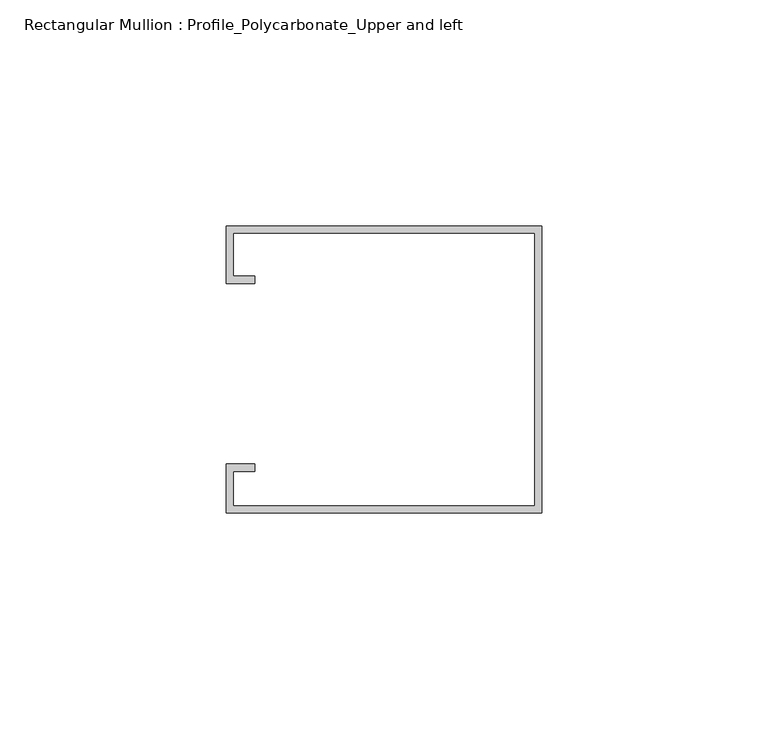
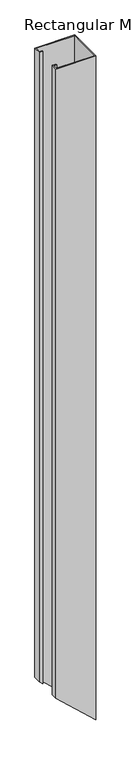
"""IFC4 building model written with IfcOpenShell, lengths in millimetres: member geometry, Rectangular Mullion : Profile_Polycarbonate_Upper and left."""

from ifc_helpers import new_model, si_unit, origin, place, context, project, spatial, faceted_brep, source, transform, mapped, element, save


def rectangular_mullion_profile_polycarbonate_upper_and_left_4dc07991(model_context):
    return source(origin(), model_context, "Body", "Brep", [
        faceted_brep([(0.0, 32.7, 0.0), (-69.85, 32.7, 0.0), (-69.85, 20.0, 0.0), (-63.5, 20.0, 0.0), (-63.5, 21.5875, 0.0), (-68.2625, 21.5875, 0.0), (-68.2625, 31.1125, 0.0), (-1.5875, 31.1125, 0.0), (-1.5875, -29.2125, 0.0), (-68.2625, -29.2125, 0.0), (-68.2625, -21.5875, 0.0), (-63.5, -21.5875, 0.0), (-63.5, -20.0, 0.0), (-69.85, -20.0, 0.0), (-69.85, -30.8, 0.0), (0.0, -30.8, 0.0), (0.0, 32.7, -1225.0208333), (-69.85, 32.7, -1160.7495516), (-69.85, 20.0, -1160.7495516), (-63.5, 20.0, -1166.5923954), (-63.5, 21.5875, -1166.5923954), (-68.2625, 21.5875, -1162.2102625), (-68.2625, 31.1125, -1162.2102625), (-1.5875, 31.1125, -1223.5601224), (-1.5875, -29.2125, -1223.5601224), (-68.2625, -29.2125, -1162.2102625), (-68.2625, -21.5875, -1162.2102625), (-63.5, -21.5875, -1166.5923954), (-63.5, -20.0, -1166.5923954), (-69.85, -20.0, -1160.7495516), (-69.85, -30.8, -1160.7495516), (0.0, -30.8, -1225.0208333)], [[[0, 1, 2, 3, 4, 5, 6, 7, 8, 9, 10, 11, 12, 13, 14, 15]], [[1, 0, 16, 17]], [[2, 1, 17, 18]], [[3, 2, 18, 19]], [[4, 3, 19, 20]], [[5, 4, 20, 21]], [[6, 5, 21, 22]], [[7, 6, 22, 23]], [[8, 7, 23, 24]], [[9, 8, 24, 25]], [[10, 9, 25, 26]], [[11, 10, 26, 27]], [[12, 11, 27, 28]], [[13, 12, 28, 29]], [[14, 13, 29, 30]], [[15, 14, 30, 31]], [[0, 15, 31, 16]], [[16, 31, 30, 29, 28, 27, 26, 25, 24, 23, 22, 21, 20, 19, 18, 17]]]),
    ])


if __name__ == "__main__":
    model = new_model("IFC4")
    model_context = context("Model", 3, world=origin())
    ifc_project = project(units=[si_unit("LENGTHUNIT", "METRE", prefix="MILLI")], contexts=[model_context])
    site = spatial("IfcSite", under=ifc_project)
    building = spatial("IfcBuilding", under=site)
    placement = place(None, origin())
    rectangular_mullion_profile_polycarbonate_upper_and_left_shape = rectangular_mullion_profile_polycarbonate_upper_and_left_4dc07991(model_context)
    element("IfcMember", 1, ObjectType="Rectangular Mullion : Profile_Polycarbonate_Upper and left", at=placement, inside=building, context=model_context, shape_type="MappedRepresentation", body=[
        mapped(rectangular_mullion_profile_polycarbonate_upper_and_left_shape, transform((0.0, 0.0, 0.0), x_axis=(1.0, 0.0, 0.0), y_axis=(0.0, 1.0, 0.0), z_axis=(0.0, 0.0, 1.0))),
    ])
    save(model, "model.ifc")

# Revit data of these elements
# Type "Rectangular Mullion : Profile_Polycarbonate_Upper and left"
#   built-in parameter 1007322 = 0.208333 (stored number, unit not read)
#   built-in parameter 1007321 = 0.00520833 (stored number, unit not read)
#   built-in parameter 1007320 = 0 (stored number, unit not read)
# Element 1 (IfcMember, "Rectangular Mullion : Profile_Polycarbonate_Upper and left")
#   Materials on its faces: "ALUMINUM PROFILE AT POLYCARBONATE PANEL"
# Materials
#   "ALUMINUM PROFILE AT POLYCARBONATE PANEL": class "Metal", colour RGB 244 244 244, transparency 0, Description = "Aluminum 6061", Cost = 0
